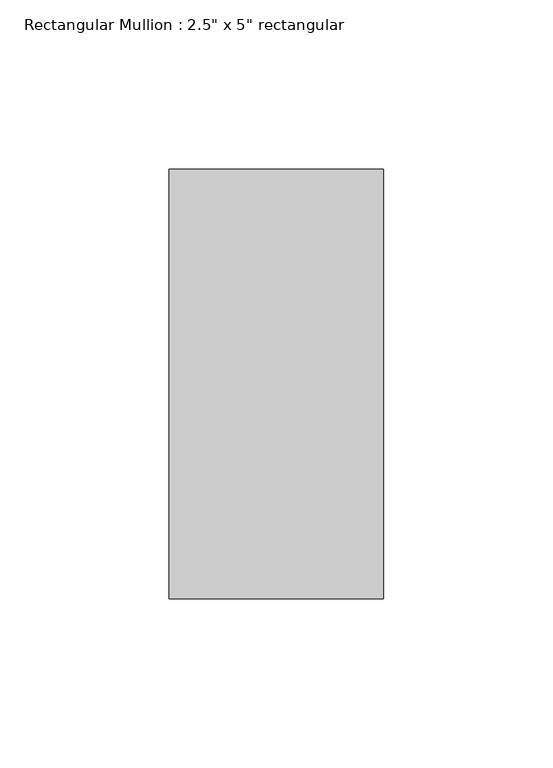
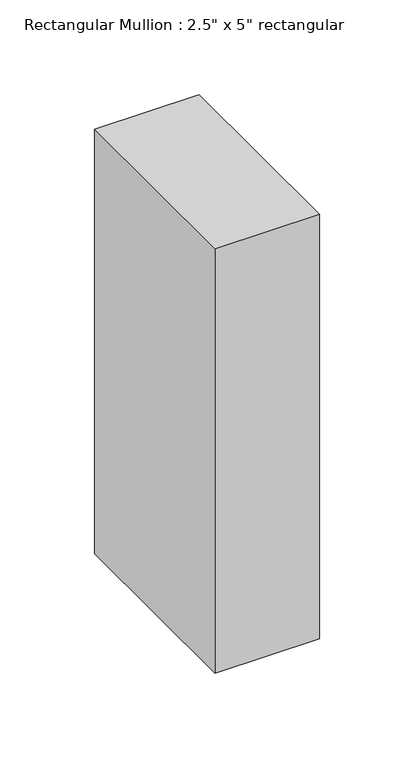
"""IFC4 building model written with IfcOpenShell, lengths in millimetres: member geometry."""

import ifcopenshell
import ifcopenshell.guid

model = None  # the IFC model being written
_history = None  # IfcOwnerHistory: only IFC2X3 demands one
_inside = {}  # id of a spatial element -> (the spatial element, [elements in it])
_under = {}  # id of a project, library or spatial element -> (it, [spatial elements below it])
_declared = {}  # id of a project -> (the project, [libraries it declares])
_typed = {}  # id of a type object -> (the type object, [elements of that type])
_made_of = {}  # id of a material, layer set ... -> (it, [elements and type objects made of it])


def new_model(schema):
    """Start an empty IFC model of exactly this schema.

    Asked for "IFC4X3", IfcOpenShell would pick the latest addendum, in which some entities
    have other attributes; the version numbers below select the first issue.
    IFC2X3 requires an IfcOwnerHistory on every rooted entity: one is made here for all.
    """
    global model, _history
    if schema == "IFC4X3":
        model = ifcopenshell.file(schema_version=(4, 3, 0, 0))
    else:
        model = ifcopenshell.file(schema=schema)
    _inside.clear()
    _under.clear()
    _declared.clear()
    _typed.clear()
    _made_of.clear()
    _history = None
    if model.schema == "IFC2X3":
        org = make("IfcOrganization", Name="unknown")
        user = make(
            "IfcPersonAndOrganization",
            ThePerson=make("IfcPerson", FamilyName="unknown"),
            TheOrganization=org,
        )
        app = make(
            "IfcApplication",
            ApplicationDeveloper=org,
            Version="unknown",
            ApplicationFullName="unknown",
            ApplicationIdentifier="unknown",
        )
        _history = make(
            "IfcOwnerHistory",
            OwningUser=user,
            OwningApplication=app,
            ChangeAction="ADDED",
            CreationDate=0,
        )
    return model


def make(cls, **values):
    """One entity of the class cls with the attributes given. An attribute that is None is left unset."""
    return model.create_entity(
        cls, **{name: value for name, value in values.items() if value is not None}
    )


def rooted(cls, **values):
    """An entity with a GlobalId (a new one), such as an element, a storey or a relation."""
    return make(cls, GlobalId=ifcopenshell.guid.new(), OwnerHistory=_history, **values)


def si_unit(unit_type, name, prefix=None):
    """IfcSIUnit, for example si_unit("LENGTHUNIT", "METRE", prefix="MILLI")."""
    return make("IfcSIUnit", UnitType=unit_type, Prefix=prefix, Name=name)


def assignment(units):
    """IfcUnitAssignment: the units of a project."""
    return None if units is None else make("IfcUnitAssignment", Units=units)


def point(xyz):
    """IfcCartesianPoint."""
    return None if xyz is None else make("IfcCartesianPoint", Coordinates=xyz)


def direction(xyz):
    """IfcDirection."""
    return None if xyz is None else make("IfcDirection", DirectionRatios=xyz)


def frame(location, z_axis=None, x_axis=None):
    """IfcAxis2Placement3D, a coordinate frame: its origin and axes. An axis left out is left unset."""
    return make(
        "IfcAxis2Placement3D",
        Location=point(location),
        Axis=direction(z_axis),
        RefDirection=direction(x_axis),
    )


def origin():
    """The frame at (0, 0, 0) with its axes left unset."""
    return frame((0.0, 0.0, 0.0))


def place(relative_to, where):
    """IfcLocalPlacement: puts the frame where relative to a parent placement (None: the world)."""
    return make(
        "IfcLocalPlacement", PlacementRelTo=relative_to, RelativePlacement=where
    )


def context(
    kind, dimensions, precision=None, world=None, true_north=None, identifier=None
):
    """IfcGeometricRepresentationContext, for example the 3D "Model" context."""
    return make(
        "IfcGeometricRepresentationContext",
        ContextIdentifier=identifier,
        ContextType=kind,
        CoordinateSpaceDimension=dimensions,
        Precision=precision,
        WorldCoordinateSystem=world,
        TrueNorth=true_north,
    )


def project(units=None, contexts=None):
    """IfcProject with its units and contexts."""
    return rooted(
        "IfcProject",
        Name="project",
        RepresentationContexts=contexts,
        UnitsInContext=assignment(units),
    )


def spatial(cls, under=None, at=None, **own):
    """A site, building, storey or space (cls), placed at a placement, below another one or the project."""
    s = rooted(cls, ObjectPlacement=at, **own)
    if under is not None:
        _under.setdefault(under.id(), (under, []))[1].append(s)
    return s


def polyline(points):
    """IfcPolyline through the points."""
    return make("IfcPolyline", Points=[point(p) for p in points])


def outline(outer, holes=None, kind="AREA"):
    """IfcArbitraryClosedProfileDef: a profile drawn as a closed curve; with holes, ...WithVoids."""
    if holes is None:
        return make("IfcArbitraryClosedProfileDef", ProfileType=kind, OuterCurve=outer)
    return make(
        "IfcArbitraryProfileDefWithVoids",
        ProfileType=kind,
        OuterCurve=outer,
        InnerCurves=holes,
    )


def extrude(swept, where, along, depth):
    """IfcExtrudedAreaSolid: the profile swept, set in the frame where, extruded along a direction by depth."""
    return make(
        "IfcExtrudedAreaSolid",
        SweptArea=swept,
        Position=where,
        ExtrudedDirection=direction(along),
        Depth=depth,
    )


def shape(context_of_items, identifier, shape_type, items):
    """IfcShapeRepresentation: the items that make up one representation, for example the "Body"."""
    return make(
        "IfcShapeRepresentation",
        ContextOfItems=context_of_items,
        RepresentationIdentifier=identifier,
        RepresentationType=shape_type,
        Items=items,
    )


def source(mapping_origin, context_of_items, identifier, shape_type, items):
    """IfcRepresentationMap: a shape defined once, which mapped items show again and again."""
    return make(
        "IfcRepresentationMap",
        MappingOrigin=mapping_origin,
        MappedRepresentation=shape(context_of_items, identifier, shape_type, items),
    )


def transform(
    local_origin,
    x_axis=None,
    y_axis=None,
    z_axis=None,
    scale=None,
    scale2=None,
    scale3=None,
    uniform=True,
):
    """IfcCartesianTransformationOperator3D, or its non-uniform kind. x_axis, y_axis, z_axis: its Axis1, 2, 3."""
    if uniform:
        return make(
            "IfcCartesianTransformationOperator3D",
            Axis1=direction(x_axis),
            Axis2=direction(y_axis),
            LocalOrigin=point(local_origin),
            Scale=scale,
            Axis3=direction(z_axis),
        )
    return make(
        "IfcCartesianTransformationOperator3DnonUniform",
        Axis1=direction(x_axis),
        Axis2=direction(y_axis),
        LocalOrigin=point(local_origin),
        Scale=scale,
        Axis3=direction(z_axis),
        Scale2=scale2,
        Scale3=scale3,
    )


def mapped(mapping_source, mapping_target):
    """IfcMappedItem: shows the shape of a source again, moved by a transform."""
    return make(
        "IfcMappedItem", MappingSource=mapping_source, MappingTarget=mapping_target
    )


def made_of(thing, what):
    """Note that an element or type object is made of a material, layer set ...; save() writes the relation."""
    if what is not None:
        _made_of.setdefault(what.id(), (what, []))[1].append(thing)
    return thing


def element(
    cls,
    number,
    at=None,
    inside=None,
    cuts=None,
    type_object=None,
    material=None,
    context=None,
    identifier="Body",
    shape_type=None,
    held_by="IfcProductDefinitionShape",
    body=None,
    shapes=None,
    **own,
):
    """One element of the class cls, such as IfcWall. Its Tag is "e" and its number.

    at: its placement. inside: the storey or other place that contains it. cuts: it is an
    opening in that element (IfcRelVoidsElement). A single representation is given by context,
    identifier, shape_type and body (its items); several are given by shapes. held_by: the class
    of the entity that holds the representations. save() writes the other relations.
    """
    e = rooted(cls, Tag="e%d" % number, ObjectPlacement=at, **own)
    if body is not None:
        shapes = [shape(context, identifier, shape_type, body)]
    if shapes is not None:
        e.Representation = make(held_by, Representations=shapes)
    if inside is not None:
        _inside.setdefault(inside.id(), (inside, []))[1].append(e)
    if cuts is not None:
        rooted(
            "IfcRelVoidsElement", RelatingBuildingElement=cuts, RelatedOpeningElement=e
        )
    if type_object is not None:
        _typed.setdefault(type_object.id(), (type_object, []))[1].append(e)
    return made_of(e, material)


def aggregate(whole, parts):
    """IfcRelAggregates: a whole, such as a stair, and the parts it consists of."""
    return rooted("IfcRelAggregates", RelatingObject=whole, RelatedObjects=parts)


def save(model, path):
    """Write the relations noted so far, then the file.

    IfcRelAggregates (storeys below a building ...), IfcRelContainedInSpatialStructure (elements
    in a storey), IfcRelDefinesByType, IfcRelAssociatesMaterial and IfcRelDeclares: one each for
    every whole, place, type object, material and project.
    """
    for whole, parts in _under.values():
        aggregate(whole, parts)
    for where, things in _inside.values():
        rooted(
            "IfcRelContainedInSpatialStructure",
            RelatedElements=things,
            RelatingStructure=where,
        )
    for kind, things in _typed.values():
        rooted("IfcRelDefinesByType", RelatedObjects=things, RelatingType=kind)
    for what, things in _made_of.values():
        rooted("IfcRelAssociatesMaterial", RelatedObjects=things, RelatingMaterial=what)
    for by, libraries in _declared.values():
        rooted("IfcRelDeclares", RelatingContext=by, RelatedDefinitions=libraries)
    model.write(path)


def member_c327c56d(model_context):
    return source(origin(), model_context, "Body", "SweptSolid", [
        extrude(outline(polyline([(0.0, 63.5), (0.0, -63.5), (-63.5, -63.5), (-63.5, 63.5), (0.0, 63.5)])), frame((0.0, 0.0, -273.05), z_axis=(0.0, 0.0, 1.0), x_axis=(1.0, 0.0, 0.0)), (0.0, 0.0, 1.0), 273.05),
    ])


if __name__ == "__main__":
    model = new_model("IFC4")
    model_context = context("Model", 3, world=origin())
    ifc_project = project(units=[si_unit("LENGTHUNIT", "METRE", prefix="MILLI")], contexts=[model_context])
    site = spatial("IfcSite", under=ifc_project)
    building = spatial("IfcBuilding", under=site)
    placement = place(None, origin())
    member_shape = member_c327c56d(model_context)
    element("IfcMember", 1, ObjectType="Rectangular Mullion : 2.5\" x 5\" rectangular", at=placement, inside=building, context=model_context, shape_type="MappedRepresentation", body=[
        mapped(member_shape, transform((0.0, 0.0, 0.0), x_axis=(1.0, 0.0, 0.0), y_axis=(0.0, 1.0, 0.0), z_axis=(0.0, 0.0, 1.0))),
    ])
    save(model, "model.ifc")

# Revit data of these elements
# Type "Rectangular Mullion : 2.5\" x 5\" rectangular"
#   built-in parameter 1007304 = 0.416667 (stored number, unit not read)
#   built-in parameter 1007301 = 0.104167 (stored number, unit not read)
#   built-in parameter 1007300 = 0.104167 (stored number, unit not read)
# Element 1 (IfcMember, "Rectangular Mullion : 2.5\" x 5\" rectangular")
#   Materials on its faces: "Metal - Aluminum"
# Materials
#   "Metal - Aluminum": class "Metal", colour RGB 140 140 140, transparency 0
